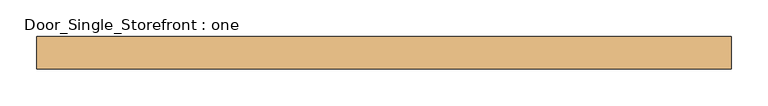
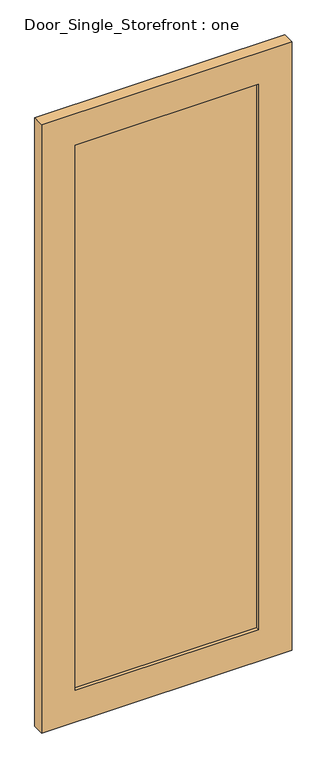
"""IFC4 building model written with IfcOpenShell, lengths in millimetres: door geometry, Door_Single_Storefront : one."""

import ifcopenshell
import ifcopenshell.guid

model = None  # the IFC model being written
_history = None  # IfcOwnerHistory: only IFC2X3 demands one
_inside = {}  # id of a spatial element -> (the spatial element, [elements in it])
_under = {}  # id of a project, library or spatial element -> (it, [spatial elements below it])
_declared = {}  # id of a project -> (the project, [libraries it declares])
_typed = {}  # id of a type object -> (the type object, [elements of that type])
_made_of = {}  # id of a material, layer set ... -> (it, [elements and type objects made of it])


def new_model(schema):
    """Start an empty IFC model of exactly this schema.

    Asked for "IFC4X3", IfcOpenShell would pick the latest addendum, in which some entities
    have other attributes; the version numbers below select the first issue.
    IFC2X3 requires an IfcOwnerHistory on every rooted entity: one is made here for all.
    """
    global model, _history
    if schema == "IFC4X3":
        model = ifcopenshell.file(schema_version=(4, 3, 0, 0))
    else:
        model = ifcopenshell.file(schema=schema)
    _inside.clear()
    _under.clear()
    _declared.clear()
    _typed.clear()
    _made_of.clear()
    _history = None
    if model.schema == "IFC2X3":
        org = make("IfcOrganization", Name="unknown")
        user = make(
            "IfcPersonAndOrganization",
            ThePerson=make("IfcPerson", FamilyName="unknown"),
            TheOrganization=org,
        )
        app = make(
            "IfcApplication",
            ApplicationDeveloper=org,
            Version="unknown",
            ApplicationFullName="unknown",
            ApplicationIdentifier="unknown",
        )
        _history = make(
            "IfcOwnerHistory",
            OwningUser=user,
            OwningApplication=app,
            ChangeAction="ADDED",
            CreationDate=0,
        )
    return model


def make(cls, **values):
    """One entity of the class cls with the attributes given. An attribute that is None is left unset."""
    return model.create_entity(
        cls, **{name: value for name, value in values.items() if value is not None}
    )


def rooted(cls, **values):
    """An entity with a GlobalId (a new one), such as an element, a storey or a relation."""
    return make(cls, GlobalId=ifcopenshell.guid.new(), OwnerHistory=_history, **values)


def si_unit(unit_type, name, prefix=None):
    """IfcSIUnit, for example si_unit("LENGTHUNIT", "METRE", prefix="MILLI")."""
    return make("IfcSIUnit", UnitType=unit_type, Prefix=prefix, Name=name)


def assignment(units):
    """IfcUnitAssignment: the units of a project."""
    return None if units is None else make("IfcUnitAssignment", Units=units)


def point(xyz):
    """IfcCartesianPoint."""
    return None if xyz is None else make("IfcCartesianPoint", Coordinates=xyz)


def direction(xyz):
    """IfcDirection."""
    return None if xyz is None else make("IfcDirection", DirectionRatios=xyz)


def frame(location, z_axis=None, x_axis=None):
    """IfcAxis2Placement3D, a coordinate frame: its origin and axes. An axis left out is left unset."""
    return make(
        "IfcAxis2Placement3D",
        Location=point(location),
        Axis=direction(z_axis),
        RefDirection=direction(x_axis),
    )


def origin():
    """The frame at (0, 0, 0) with its axes left unset."""
    return frame((0.0, 0.0, 0.0))


def place(relative_to, where):
    """IfcLocalPlacement: puts the frame where relative to a parent placement (None: the world)."""
    return make(
        "IfcLocalPlacement", PlacementRelTo=relative_to, RelativePlacement=where
    )


def context(
    kind, dimensions, precision=None, world=None, true_north=None, identifier=None
):
    """IfcGeometricRepresentationContext, for example the 3D "Model" context."""
    return make(
        "IfcGeometricRepresentationContext",
        ContextIdentifier=identifier,
        ContextType=kind,
        CoordinateSpaceDimension=dimensions,
        Precision=precision,
        WorldCoordinateSystem=world,
        TrueNorth=true_north,
    )


def project(units=None, contexts=None):
    """IfcProject with its units and contexts."""
    return rooted(
        "IfcProject",
        Name="project",
        RepresentationContexts=contexts,
        UnitsInContext=assignment(units),
    )


def spatial(cls, under=None, at=None, **own):
    """A site, building, storey or space (cls), placed at a placement, below another one or the project."""
    s = rooted(cls, ObjectPlacement=at, **own)
    if under is not None:
        _under.setdefault(under.id(), (under, []))[1].append(s)
    return s


def polyline(points):
    """IfcPolyline through the points."""
    return make("IfcPolyline", Points=[point(p) for p in points])


def outline(outer, holes=None, kind="AREA"):
    """IfcArbitraryClosedProfileDef: a profile drawn as a closed curve; with holes, ...WithVoids."""
    if holes is None:
        return make("IfcArbitraryClosedProfileDef", ProfileType=kind, OuterCurve=outer)
    return make(
        "IfcArbitraryProfileDefWithVoids",
        ProfileType=kind,
        OuterCurve=outer,
        InnerCurves=holes,
    )


def extrude(swept, where, along, depth):
    """IfcExtrudedAreaSolid: the profile swept, set in the frame where, extruded along a direction by depth."""
    return make(
        "IfcExtrudedAreaSolid",
        SweptArea=swept,
        Position=where,
        ExtrudedDirection=direction(along),
        Depth=depth,
    )


def shape(context_of_items, identifier, shape_type, items):
    """IfcShapeRepresentation: the items that make up one representation, for example the "Body"."""
    return make(
        "IfcShapeRepresentation",
        ContextOfItems=context_of_items,
        RepresentationIdentifier=identifier,
        RepresentationType=shape_type,
        Items=items,
    )


def source(mapping_origin, context_of_items, identifier, shape_type, items):
    """IfcRepresentationMap: a shape defined once, which mapped items show again and again."""
    return make(
        "IfcRepresentationMap",
        MappingOrigin=mapping_origin,
        MappedRepresentation=shape(context_of_items, identifier, shape_type, items),
    )


def transform(
    local_origin,
    x_axis=None,
    y_axis=None,
    z_axis=None,
    scale=None,
    scale2=None,
    scale3=None,
    uniform=True,
):
    """IfcCartesianTransformationOperator3D, or its non-uniform kind. x_axis, y_axis, z_axis: its Axis1, 2, 3."""
    if uniform:
        return make(
            "IfcCartesianTransformationOperator3D",
            Axis1=direction(x_axis),
            Axis2=direction(y_axis),
            LocalOrigin=point(local_origin),
            Scale=scale,
            Axis3=direction(z_axis),
        )
    return make(
        "IfcCartesianTransformationOperator3DnonUniform",
        Axis1=direction(x_axis),
        Axis2=direction(y_axis),
        LocalOrigin=point(local_origin),
        Scale=scale,
        Axis3=direction(z_axis),
        Scale2=scale2,
        Scale3=scale3,
    )


def mapped(mapping_source, mapping_target):
    """IfcMappedItem: shows the shape of a source again, moved by a transform."""
    return make(
        "IfcMappedItem", MappingSource=mapping_source, MappingTarget=mapping_target
    )


def made_of(thing, what):
    """Note that an element or type object is made of a material, layer set ...; save() writes the relation."""
    if what is not None:
        _made_of.setdefault(what.id(), (what, []))[1].append(thing)
    return thing


def element(
    cls,
    number,
    at=None,
    inside=None,
    cuts=None,
    type_object=None,
    material=None,
    context=None,
    identifier="Body",
    shape_type=None,
    held_by="IfcProductDefinitionShape",
    body=None,
    shapes=None,
    **own,
):
    """One element of the class cls, such as IfcWall. Its Tag is "e" and its number.

    at: its placement. inside: the storey or other place that contains it. cuts: it is an
    opening in that element (IfcRelVoidsElement). A single representation is given by context,
    identifier, shape_type and body (its items); several are given by shapes. held_by: the class
    of the entity that holds the representations. save() writes the other relations.
    """
    e = rooted(cls, Tag="e%d" % number, ObjectPlacement=at, **own)
    if body is not None:
        shapes = [shape(context, identifier, shape_type, body)]
    if shapes is not None:
        e.Representation = make(held_by, Representations=shapes)
    if inside is not None:
        _inside.setdefault(inside.id(), (inside, []))[1].append(e)
    if cuts is not None:
        rooted(
            "IfcRelVoidsElement", RelatingBuildingElement=cuts, RelatedOpeningElement=e
        )
    if type_object is not None:
        _typed.setdefault(type_object.id(), (type_object, []))[1].append(e)
    return made_of(e, material)


def aggregate(whole, parts):
    """IfcRelAggregates: a whole, such as a stair, and the parts it consists of."""
    return rooted("IfcRelAggregates", RelatingObject=whole, RelatedObjects=parts)


def save(model, path):
    """Write the relations noted so far, then the file.

    IfcRelAggregates (storeys below a building ...), IfcRelContainedInSpatialStructure (elements
    in a storey), IfcRelDefinesByType, IfcRelAssociatesMaterial and IfcRelDeclares: one each for
    every whole, place, type object, material and project.
    """
    for whole, parts in _under.values():
        aggregate(whole, parts)
    for where, things in _inside.values():
        rooted(
            "IfcRelContainedInSpatialStructure",
            RelatedElements=things,
            RelatingStructure=where,
        )
    for kind, things in _typed.values():
        rooted("IfcRelDefinesByType", RelatedObjects=things, RelatingType=kind)
    for what, things in _made_of.values():
        rooted("IfcRelAssociatesMaterial", RelatedObjects=things, RelatingMaterial=what)
    for by, libraries in _declared.values():
        rooted("IfcRelDeclares", RelatingContext=by, RelatedDefinitions=libraries)
    model.write(path)


def door_single_storefront_one_36bbcdfe(model_context):
    return source(origin(), model_context, "Body", "SweptSolid", [
        extrude(outline(polyline([(347.6625, -6.35), (-347.6625, -6.35), (-347.6625, 12.7), (347.6625, 12.7), (347.6625, -6.35)])), frame((0.0, 0.0, 127.0), z_axis=(0.0, 0.0, 1.0), x_axis=(1.0, 0.0, 0.0)), (0.0, 0.0, 1.0), 2184.4),
        extrude(outline(polyline([(2438.4, -474.6625), (0.0, -474.6625), (0.0, 474.6625), (2438.4, 474.6625), (2438.4, -474.6625)]), holes=[polyline([(127.0, 347.6625), (127.0, -347.6625), (2311.4, -347.6625), (2311.4, 347.6625), (127.0, 347.6625)])]), frame((0.0, -19.05, 0.0), z_axis=(0.0, 1.0, 0.0), x_axis=(0.0, 0.0, 1.0)), (0.0, 0.0, 1.0), 44.45),
    ])


if __name__ == "__main__":
    model = new_model("IFC4")
    model_context = context("Model", 3, world=origin())
    ifc_project = project(units=[si_unit("LENGTHUNIT", "METRE", prefix="MILLI")], contexts=[model_context])
    site = spatial("IfcSite", under=ifc_project)
    building = spatial("IfcBuilding", under=site)
    placement = place(None, origin())
    door_single_storefront_one_shape = door_single_storefront_one_36bbcdfe(model_context)
    element("IfcDoor", 1, ObjectType="Door_Single_Storefront : one", at=placement, inside=building, context=model_context, shape_type="MappedRepresentation", body=[
        mapped(door_single_storefront_one_shape, transform((0.0, 0.0, 0.0), x_axis=(1.0, 0.0, 0.0), y_axis=(0.0, 1.0, 0.0), z_axis=(0.0, 0.0, 1.0))),
    ])
    save(model, "model.ifc")

# Revit data of these elements
# Type "Door_Single_Storefront : one"
#   Type Mark = "27"
#   Analytic Construction = "<None>"
#   Stile_Width = 0' - 5"
#   Door_Thickness = 0' - 1 3/4"
#   Door_Offset = 0' - 1"
#   Glass_Material = SAFETY GLAZING
#   Frame_Material = INTERIOR GRADE ALUMINUM STOREFRONT W/ SAFETY GLAZING
#   Function = (empty or 0)
# Element 1 (IfcDoor, "Door_Single_Storefront : one")
#   Materials on its faces: "INTERIOR GRADE ALUMINUM STOREFRONT W/ SAFETY GLAZING", "SAFETY GLAZING"
# Materials
#   "SAFETY GLAZING": class "Glass", colour RGB 142 168 196, transparency 0.75, Description = "Soda Lime Glass", Cost = 0
#   "INTERIOR GRADE ALUMINUM STOREFRONT W/ SAFETY GLAZING": class "Metal", colour RGB 226 226 226, transparency 0, Description = "Aluminum 6061", Cost = 0
